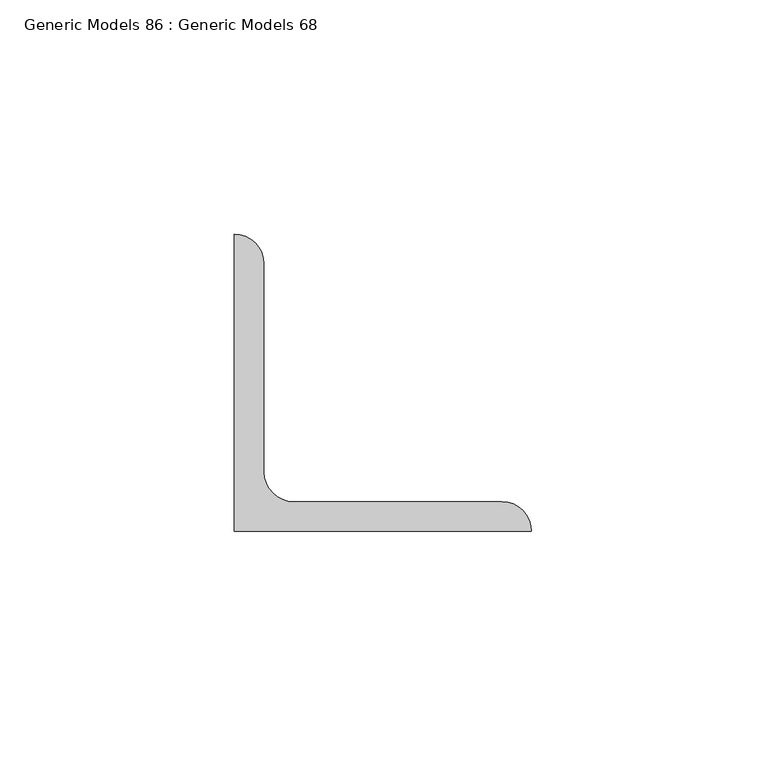
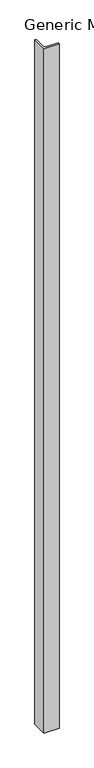
"""IFC4 building model written with IfcOpenShell, lengths in millimetres: proxy geometry, Generic Models 86 : Generic Models 68."""

from ifc_helpers import new_model, si_unit, point, frame, frame_2d, origin, place, context, project, spatial, polyline, circle_curve, trimmed, segment, composite_curve, outline, extrude, source, transform, mapped, element, save


def generic_models_86_generic_models_68_c7985be7(model_context):
    return source(origin(), model_context, "Body", "SweptSolid", [
        extrude(outline(composite_curve([segment(polyline([(20530.4116945, 20934.4264581), (20530.4116945, 20997.9264581)]), True, "CONTINUOUS"), segment(trimmed(circle_curve(frame_2d((20530.4116945, 20991.5764581)), 6.35), [point((20530.4116945, 20997.9264581))], [point((20536.7616945, 20991.5764581))], False, "CARTESIAN"), True, "CONTINUOUS"), segment(polyline([(20536.7616945, 20991.5764581), (20536.7616945, 20947.1264581)]), True, "CONTINUOUS"), segment(trimmed(circle_curve(frame_2d((20543.1116945, 20947.1264581)), 6.35), [point((20536.7616945, 20947.1264581))], [point((20543.1116945, 20940.7764581))], True, "CARTESIAN"), True, "CONTINUOUS"), segment(polyline([(20543.1116945, 20940.7764581), (20587.5616945, 20940.7764581)]), True, "CONTINUOUS"), segment(trimmed(circle_curve(frame_2d((20587.5616945, 20934.4264581)), 6.35), [point((20587.5616945, 20940.7764581))], [point((20593.9116945, 20934.4264581))], False, "CARTESIAN"), True, "CONTINUOUS"), segment(polyline([(20593.9116945, 20934.4264581), (20530.4116945, 20934.4264581)]), True, "CONTINUOUS")], self_intersect=False)), frame((0.0, 0.0, 264380.6186948), z_axis=(0.0, 0.0, 1.0), x_axis=(1.0, 0.0, 0.0)), (0.0, 0.0, 1.0), 3006.09),
    ])


if __name__ == "__main__":
    model = new_model("IFC4")
    model_context = context("Model", 3, world=origin())
    ifc_project = project(units=[si_unit("LENGTHUNIT", "METRE", prefix="MILLI")], contexts=[model_context])
    site = spatial("IfcSite", under=ifc_project)
    building = spatial("IfcBuilding", under=site)
    placement = place(None, origin())
    generic_models_86_generic_models_68_shape = generic_models_86_generic_models_68_c7985be7(model_context)
    element("IfcBuildingElementProxy", 1, Name="Generic Models 86 : Generic Models 68", ObjectType="Generic Models 86 : Generic Models 68", at=placement, inside=building, context=model_context, shape_type="MappedRepresentation", body=[
        mapped(generic_models_86_generic_models_68_shape, transform((0.0, 0.0, 0.0), x_axis=(1.0, 0.0, 0.0), y_axis=(0.0, 1.0, 0.0), z_axis=(0.0, 0.0, 1.0))),
    ])
    save(model, "model.ifc")

# Revit data of these elements
# Element 1 (IfcBuildingElementProxy, "Generic Models 86 : Generic Models 68")
#   Materials on its faces: "MAIN FENCE POST: (2) BACK/BACK GALVANIZED ANGLES (2) L2 1/2 X 2 1/2 X 1/4\") ANCHORED TO 8\"W X 42\" DEEP CONCRETE FOOTING(1)"
# Materials
#   "MAIN FENCE POST: (2) BACK/BACK GALVANIZED ANGLES (2) L2 1/2 X 2 1/2 X 1/4\") ANCHORED TO 8\"W X 42\" DEEP CONCRETE FOOTING(1)": class "Unassigned", colour RGB 211 211 211, transparency 0, Cost = 0
